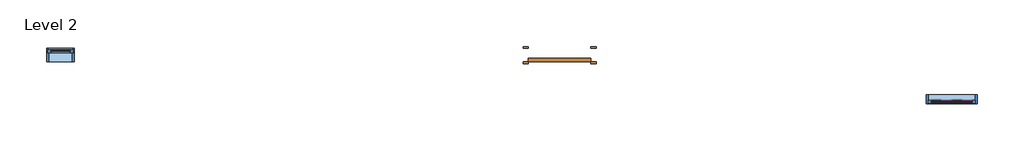
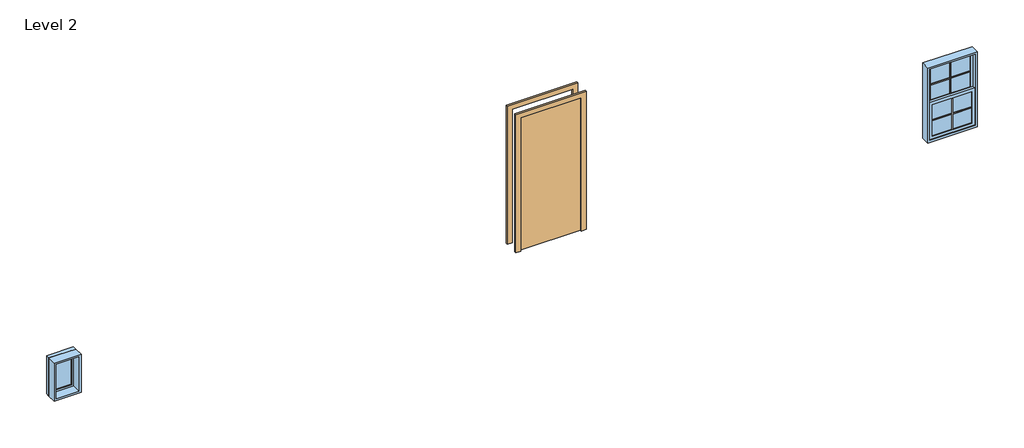
# One storey: 2 proxies, 2 windows, 1 door.
"""IFC4 building model written with IfcOpenShell, lengths in millimetres."""

import ifcopenshell
import ifcopenshell.guid

model = None  # the IFC model being written
_history = None  # IfcOwnerHistory: only IFC2X3 demands one
_inside = {}  # id of a spatial element -> (the spatial element, [elements in it])
_under = {}  # id of a project, library or spatial element -> (it, [spatial elements below it])
_declared = {}  # id of a project -> (the project, [libraries it declares])
_typed = {}  # id of a type object -> (the type object, [elements of that type])
_made_of = {}  # id of a material, layer set ... -> (it, [elements and type objects made of it])


def new_model(schema):
    """Start an empty IFC model of exactly this schema.

    Asked for "IFC4X3", IfcOpenShell would pick the latest addendum, in which some entities
    have other attributes; the version numbers below select the first issue.
    IFC2X3 requires an IfcOwnerHistory on every rooted entity: one is made here for all.
    """
    global model, _history
    if schema == "IFC4X3":
        model = ifcopenshell.file(schema_version=(4, 3, 0, 0))
    else:
        model = ifcopenshell.file(schema=schema)
    _inside.clear()
    _under.clear()
    _declared.clear()
    _typed.clear()
    _made_of.clear()
    _history = None
    if model.schema == "IFC2X3":
        org = make("IfcOrganization", Name="unknown")
        user = make(
            "IfcPersonAndOrganization",
            ThePerson=make("IfcPerson", FamilyName="unknown"),
            TheOrganization=org,
        )
        app = make(
            "IfcApplication",
            ApplicationDeveloper=org,
            Version="unknown",
            ApplicationFullName="unknown",
            ApplicationIdentifier="unknown",
        )
        _history = make(
            "IfcOwnerHistory",
            OwningUser=user,
            OwningApplication=app,
            ChangeAction="ADDED",
            CreationDate=0,
        )
    return model


def make(cls, **values):
    """One entity of the class cls with the attributes given. An attribute that is None is left unset."""
    return model.create_entity(
        cls, **{name: value for name, value in values.items() if value is not None}
    )


def rooted(cls, **values):
    """An entity with a GlobalId (a new one), such as an element, a storey or a relation."""
    return make(cls, GlobalId=ifcopenshell.guid.new(), OwnerHistory=_history, **values)


def si_unit(unit_type, name, prefix=None):
    """IfcSIUnit, for example si_unit("LENGTHUNIT", "METRE", prefix="MILLI")."""
    return make("IfcSIUnit", UnitType=unit_type, Prefix=prefix, Name=name)


def assignment(units):
    """IfcUnitAssignment: the units of a project."""
    return None if units is None else make("IfcUnitAssignment", Units=units)


def point(xyz):
    """IfcCartesianPoint."""
    return None if xyz is None else make("IfcCartesianPoint", Coordinates=xyz)


def direction(xyz):
    """IfcDirection."""
    return None if xyz is None else make("IfcDirection", DirectionRatios=xyz)


def frame(location, z_axis=None, x_axis=None):
    """IfcAxis2Placement3D, a coordinate frame: its origin and axes. An axis left out is left unset."""
    return make(
        "IfcAxis2Placement3D",
        Location=point(location),
        Axis=direction(z_axis),
        RefDirection=direction(x_axis),
    )


def origin():
    """The frame at (0, 0, 0) with its axes left unset."""
    return frame((0.0, 0.0, 0.0))


def origin_with_axes():
    """The frame at (0, 0, 0) with the z axis (0, 0, 1) and the x axis (1, 0, 0) written out."""
    return frame((0.0, 0.0, 0.0), z_axis=(0.0, 0.0, 1.0), x_axis=(1.0, 0.0, 0.0))


def place(relative_to, where):
    """IfcLocalPlacement: puts the frame where relative to a parent placement (None: the world)."""
    return make(
        "IfcLocalPlacement", PlacementRelTo=relative_to, RelativePlacement=where
    )


def context(
    kind, dimensions, precision=None, world=None, true_north=None, identifier=None
):
    """IfcGeometricRepresentationContext, for example the 3D "Model" context."""
    return make(
        "IfcGeometricRepresentationContext",
        ContextIdentifier=identifier,
        ContextType=kind,
        CoordinateSpaceDimension=dimensions,
        Precision=precision,
        WorldCoordinateSystem=world,
        TrueNorth=true_north,
    )


def project(units=None, contexts=None):
    """IfcProject with its units and contexts."""
    return rooted(
        "IfcProject",
        Name="project",
        RepresentationContexts=contexts,
        UnitsInContext=assignment(units),
    )


def spatial(cls, under=None, at=None, **own):
    """A site, building, storey or space (cls), placed at a placement, below another one or the project."""
    s = rooted(cls, ObjectPlacement=at, **own)
    if under is not None:
        _under.setdefault(under.id(), (under, []))[1].append(s)
    return s


def polyline(points):
    """IfcPolyline through the points."""
    return make("IfcPolyline", Points=[point(p) for p in points])


def outline(outer, holes=None, kind="AREA"):
    """IfcArbitraryClosedProfileDef: a profile drawn as a closed curve; with holes, ...WithVoids."""
    if holes is None:
        return make("IfcArbitraryClosedProfileDef", ProfileType=kind, OuterCurve=outer)
    return make(
        "IfcArbitraryProfileDefWithVoids",
        ProfileType=kind,
        OuterCurve=outer,
        InnerCurves=holes,
    )


def extrude(swept, where, along, depth):
    """IfcExtrudedAreaSolid: the profile swept, set in the frame where, extruded along a direction by depth."""
    return make(
        "IfcExtrudedAreaSolid",
        SweptArea=swept,
        Position=where,
        ExtrudedDirection=direction(along),
        Depth=depth,
    )


def shape(context_of_items, identifier, shape_type, items):
    """IfcShapeRepresentation: the items that make up one representation, for example the "Body"."""
    return make(
        "IfcShapeRepresentation",
        ContextOfItems=context_of_items,
        RepresentationIdentifier=identifier,
        RepresentationType=shape_type,
        Items=items,
    )


def source(mapping_origin, context_of_items, identifier, shape_type, items):
    """IfcRepresentationMap: a shape defined once, which mapped items show again and again."""
    return make(
        "IfcRepresentationMap",
        MappingOrigin=mapping_origin,
        MappedRepresentation=shape(context_of_items, identifier, shape_type, items),
    )


def transform(
    local_origin,
    x_axis=None,
    y_axis=None,
    z_axis=None,
    scale=None,
    scale2=None,
    scale3=None,
    uniform=True,
):
    """IfcCartesianTransformationOperator3D, or its non-uniform kind. x_axis, y_axis, z_axis: its Axis1, 2, 3."""
    if uniform:
        return make(
            "IfcCartesianTransformationOperator3D",
            Axis1=direction(x_axis),
            Axis2=direction(y_axis),
            LocalOrigin=point(local_origin),
            Scale=scale,
            Axis3=direction(z_axis),
        )
    return make(
        "IfcCartesianTransformationOperator3DnonUniform",
        Axis1=direction(x_axis),
        Axis2=direction(y_axis),
        LocalOrigin=point(local_origin),
        Scale=scale,
        Axis3=direction(z_axis),
        Scale2=scale2,
        Scale3=scale3,
    )


def mapped(mapping_source, mapping_target):
    """IfcMappedItem: shows the shape of a source again, moved by a transform."""
    return make(
        "IfcMappedItem", MappingSource=mapping_source, MappingTarget=mapping_target
    )


def made_of(thing, what):
    """Note that an element or type object is made of a material, layer set ...; save() writes the relation."""
    if what is not None:
        _made_of.setdefault(what.id(), (what, []))[1].append(thing)
    return thing


def element(
    cls,
    number,
    at=None,
    inside=None,
    cuts=None,
    type_object=None,
    material=None,
    context=None,
    identifier="Body",
    shape_type=None,
    held_by="IfcProductDefinitionShape",
    body=None,
    shapes=None,
    **own,
):
    """One element of the class cls, such as IfcWall. Its Tag is "e" and its number.

    at: its placement. inside: the storey or other place that contains it. cuts: it is an
    opening in that element (IfcRelVoidsElement). A single representation is given by context,
    identifier, shape_type and body (its items); several are given by shapes. held_by: the class
    of the entity that holds the representations. save() writes the other relations.
    """
    e = rooted(cls, Tag="e%d" % number, ObjectPlacement=at, **own)
    if body is not None:
        shapes = [shape(context, identifier, shape_type, body)]
    if shapes is not None:
        e.Representation = make(held_by, Representations=shapes)
    if inside is not None:
        _inside.setdefault(inside.id(), (inside, []))[1].append(e)
    if cuts is not None:
        rooted(
            "IfcRelVoidsElement", RelatingBuildingElement=cuts, RelatedOpeningElement=e
        )
    if type_object is not None:
        _typed.setdefault(type_object.id(), (type_object, []))[1].append(e)
    return made_of(e, material)


def aggregate(whole, parts):
    """IfcRelAggregates: a whole, such as a stair, and the parts it consists of."""
    return rooted("IfcRelAggregates", RelatingObject=whole, RelatedObjects=parts)


def save(model, path):
    """Write the relations noted so far, then the file.

    IfcRelAggregates (storeys below a building ...), IfcRelContainedInSpatialStructure (elements
    in a storey), IfcRelDefinesByType, IfcRelAssociatesMaterial and IfcRelDeclares: one each for
    every whole, place, type object, material and project.
    """
    for whole, parts in _under.values():
        aggregate(whole, parts)
    for where, things in _inside.values():
        rooted(
            "IfcRelContainedInSpatialStructure",
            RelatedElements=things,
            RelatingStructure=where,
        )
    for kind, things in _typed.values():
        rooted("IfcRelDefinesByType", RelatedObjects=things, RelatingType=kind)
    for what, things in _made_of.values():
        rooted("IfcRelAssociatesMaterial", RelatedObjects=things, RelatingMaterial=what)
    for by, libraries in _declared.values():
        rooted("IfcRelDeclares", RelatingContext=by, RelatedDefinitions=libraries)
    model.write(path)


def m_muntin_pattern_2x2_m_muntin_pattern_2x2_aaec3afb(model_context):
    return source(origin(), model_context, "Body", "SweptSolid", [
        extrude(outline(polyline([(257.1375, -6.35), (257.1375, -298.8), (244.4375, -298.8), (244.4375, -6.35), (0.0, -6.35), (0.0, 6.35), (244.4375, 6.35), (244.4375, 298.8), (257.1375, 298.8), (257.1375, 6.35), (501.575, 6.35), (501.575, -6.35), (257.1375, -6.35)])), frame((0.0, 9.525, 0.0), z_axis=(0.0, 1.0, 0.0), x_axis=(0.0, 0.0, 1.0)), (0.0, 0.0, 1.0), 12.7),
        extrude(outline(polyline([(257.1375, -6.35), (257.1375, -298.8), (244.4375, -298.8), (244.4375, -6.35), (0.0, -6.35), (0.0, 6.35), (244.4375, 6.35), (244.4375, 298.8), (257.1375, 298.8), (257.1375, 6.35), (501.575, 6.35), (501.575, -6.35), (257.1375, -6.35)])), frame((0.0, -22.225, 0.0), z_axis=(0.0, 1.0, 0.0), x_axis=(0.0, 0.0, 1.0)), (0.0, 0.0, 1.0), 12.7),
    ])


def m_single_flush_0915_x_2134mm_6a9e8738(model_context):
    return source(origin(), model_context, "Body", "SweptSolid", [
        extrude(outline(polyline([(2210.0, -533.5), (0.0, -533.5), (0.0, -457.5), (2134.0, -457.5), (2134.0, 457.5), (0.0, 457.5), (0.0, 533.5), (2210.0, 533.5), (2210.0, -533.5)])), frame((0.0, 100.0, 0.0), z_axis=(0.0, 1.0, 0.0), x_axis=(0.0, 0.0, 1.0)), (0.0, 0.0, 1.0), 25.0),
        extrude(outline(polyline([(2210.0, 533.5), (2210.0, -533.5), (0.0, -533.5), (0.0, -457.5), (2134.0, -457.5), (2134.0, 457.5), (0.0, 457.5), (0.0, 533.5), (2210.0, 533.5)])), frame((0.0, -125.0, 0.0), z_axis=(0.0, 1.0, 0.0), x_axis=(0.0, 0.0, 1.0)), (0.0, 0.0, 1.0), 25.0),
        extrude(outline(polyline([(457.5, 49.0), (-457.5, 49.0), (-457.5, 100.0), (457.5, 100.0), (457.5, 49.0)])), origin_with_axes(), (0.0, 0.0, 1.0), 2134.0),
    ])


def m_fixed_0406_x_0610mm_8205b201(model_context):
    return source(origin(), model_context, "Body", "SweptSolid", [
        extrude(outline(polyline([(-140.0, 78.0), (140.0, 78.0), (140.0, 66.0), (-140.0, 66.0), (-140.0, 78.0)])), frame((0.0, 0.0, 978.0), z_axis=(0.0, 0.0, 1.0), x_axis=(1.0, 0.0, 0.0)), (0.0, 0.0, 1.0), 484.0),
        extrude(outline(polyline([(1506.0, -184.0), (934.0, -184.0), (934.0, 184.0), (1506.0, 184.0), (1506.0, -184.0)]), holes=[polyline([(1462.0, -140.0), (1462.0, 140.0), (978.0, 140.0), (978.0, -140.0), (1462.0, -140.0)])]), frame((0.0, 50.0, 0.0), z_axis=(0.0, 1.0, 0.0), x_axis=(0.0, 0.0, 1.0)), (0.0, 0.0, 1.0), 44.0),
        extrude(outline(polyline([(1525.0, -203.0), (915.0, -203.0), (915.0, 203.0), (1525.0, 203.0), (1525.0, -203.0)]), holes=[polyline([(1506.0, -184.0), (1506.0, 184.0), (934.0, 184.0), (934.0, -184.0), (1506.0, -184.0)])]), frame((0.0, 50.0, 0.0), z_axis=(0.0, 1.0, 0.0), x_axis=(0.0, 0.0, 1.0)), (0.0, 0.0, 1.0), 63.0),
        extrude(outline(polyline([(1525.0, -203.0), (915.0, -203.0), (915.0, 203.0), (1525.0, 203.0), (1525.0, -203.0)]), holes=[polyline([(1493.0, -171.0), (1493.0, 171.0), (947.0, 171.0), (947.0, -171.0), (1493.0, -171.0)])]), frame((0.0, -87.0, 0.0), z_axis=(0.0, 1.0, 0.0), x_axis=(0.0, 0.0, 1.0)), (0.0, 0.0, 1.0), 137.0),
    ])


def m_window_double_hung_750_x_1200mm_e7ea5f28(model_context):
    return source(origin(), model_context, "Body", "SweptSolid", [
        extrude(outline(polyline([(298.8, -669.85), (298.8, -676.2), (-298.8, -676.2), (-298.8, -669.85), (298.8, -669.85)])), frame((0.0, 0.0, 990.6), z_axis=(0.0, 0.0, 1.0), x_axis=(1.0, 0.0, 0.0)), (0.0, 0.0, 1.0), 501.575),
        extrude(outline(polyline([(-298.8, -682.55), (298.8, -682.55), (298.8, -688.9), (-298.8, -688.9), (-298.8, -682.55)])), frame((0.0, 0.0, 990.6), z_axis=(0.0, 0.0, 1.0), x_axis=(1.0, 0.0, 0.0)), (0.0, 0.0, 1.0), 501.575),
        extrude(outline(polyline([(298.8, -625.4), (298.8, -631.75), (-298.8, -631.75), (-298.8, -625.4), (298.8, -625.4)])), frame((0.0, 0.0, 1536.625), z_axis=(0.0, 0.0, 1.0), x_axis=(1.0, 0.0, 0.0)), (0.0, 0.0, 1.0), 501.575),
        extrude(outline(polyline([(-298.8, -638.1), (298.8, -638.1), (298.8, -644.45), (-298.8, -644.45), (-298.8, -638.1)])), frame((0.0, 0.0, 1536.625), z_axis=(0.0, 0.0, 1.0), x_axis=(1.0, 0.0, 0.0)), (0.0, 0.0, 1.0), 501.575),
        extrude(outline(polyline([(1536.625, -343.25), (946.15, -343.25), (946.15, 343.25), (1536.625, 343.25), (1536.625, -343.25)]), holes=[polyline([(1492.175, 298.8), (990.6, 298.8), (990.6, -298.8), (1492.175, -298.8), (1492.175, 298.8)])]), frame((0.0, -701.6, 0.0), z_axis=(0.0, 1.0, 0.0), x_axis=(0.0, 0.0, 1.0)), (0.0, 0.0, 1.0), 44.45),
        extrude(outline(polyline([(2082.65, -343.25), (1492.175, -343.25), (1492.175, 343.25), (2082.65, 343.25), (2082.65, -343.25)]), holes=[polyline([(2038.2, 298.8), (1536.625, 298.8), (1536.625, -298.8), (2038.2, -298.8), (2038.2, 298.8)])]), frame((0.0, -657.15, 0.0), z_axis=(0.0, 1.0, 0.0), x_axis=(0.0, 0.0, 1.0)), (0.0, 0.0, 1.0), 44.45),
        extrude(outline(polyline([(2114.4, -375.0), (914.4, -375.0), (914.4, 375.0), (2114.4, 375.0), (2114.4, -375.0)]), holes=[polyline([(2082.65, 343.25), (946.15, 343.25), (946.15, -343.25), (2082.65, -343.25), (2082.65, 343.25)])]), frame((0.0, -714.3, 0.0), z_axis=(0.0, 1.0, 0.0), x_axis=(0.0, 0.0, 1.0)), (0.0, 0.0, 1.0), 133.35),
    ])


model = new_model("IFC4")

# Units and contexts
model_context = context("Model", 3, world=origin())
ifc_project = project(units=[si_unit("LENGTHUNIT", "METRE", prefix="MILLI")], contexts=[model_context])

# Site, building, storey
site = spatial("IfcSite", under=ifc_project)
building = spatial("IfcBuilding", under=site)
storey = spatial("IfcBuildingStorey", under=building, Name="Level 2", Elevation=4000.0)

# Proxies
placement = place(None, origin())
m_muntin_pattern_2x2_m_muntin_pattern_2x2_shape = m_muntin_pattern_2x2_m_muntin_pattern_2x2_aaec3afb(model_context)
element("IfcBuildingElementProxy", 1, Name="M_Muntin Pattern_2x2 : M_Muntin Pattern_2x2", ObjectType="M_Muntin Pattern_2x2 : M_Muntin Pattern_2x2", at=placement, inside=storey, context=model_context, shape_type="MappedRepresentation", body=[
    mapped(m_muntin_pattern_2x2_m_muntin_pattern_2x2_shape, transform((-15264.9853759, 1399.5505832, 5536.625), x_axis=(1.0, 0.0, 0.0), y_axis=(0.0, 1.0, 0.0), z_axis=(0.0, 0.0, 1.0))),
])
element("IfcBuildingElementProxy", 2, Name="M_Muntin Pattern_2x2 : M_Muntin Pattern_2x2", ObjectType="M_Muntin Pattern_2x2 : M_Muntin Pattern_2x2", at=placement, inside=storey, context=model_context, shape_type="MappedRepresentation", body=[
    mapped(m_muntin_pattern_2x2_m_muntin_pattern_2x2_shape, transform((-15264.9853759, 1355.1005832, 4990.6), x_axis=(1.0, 0.0, 0.0), y_axis=(0.0, 1.0, 0.0), z_axis=(0.0, 0.0, 1.0))),
])

# Door
m_single_flush_0915_x_2134mm_shape = m_single_flush_0915_x_2134mm_6a9e8738(model_context)
element("IfcDoor", 3, ObjectType="M_Single-Flush : 0915 x 2134mm", at=placement, inside=storey, context=model_context, shape_type="MappedRepresentation", body=[
    mapped(m_single_flush_0915_x_2134mm_shape, transform((-20997.4853759, 2034.4755832, 4866.0), x_axis=(-1.0, 0.0, 0.0), y_axis=(0.0, -1.0, 0.0), z_axis=(0.0, 0.0, 1.0))),
])

# Windows
m_fixed_0406_x_0610mm_shape = m_fixed_0406_x_0610mm_8205b201(model_context)
element("IfcWindow", 4, ObjectType="M_Fixed : 0406 x 0610mm", at=placement, inside=storey, context=model_context, shape_type="MappedRepresentation", body=[
    mapped(m_fixed_0406_x_0610mm_shape, transform((-28293.5284847, 2021.4755832, 4000.0), x_axis=(1.0, 0.0, 0.0), y_axis=(0.0, 1.0, 0.0), z_axis=(0.0, 0.0, 1.0))),
])
m_window_double_hung_750_x_1200mm_shape = m_window_double_hung_750_x_1200mm_e7ea5f28(model_context)
element("IfcWindow", 5, ObjectType="M_Window-Double-Hung : 750 x 1200mm", at=placement, inside=storey, context=model_context, shape_type="MappedRepresentation", body=[
    mapped(m_window_double_hung_750_x_1200mm_shape, transform((-15264.9853759, 2034.4755832, 4000.0), x_axis=(1.0, 0.0, 0.0), y_axis=(0.0, 1.0, 0.0), z_axis=(0.0, 0.0, 1.0))),
])

save(model, "model.ifc")

# Revit data of these elements
# Type "M_Muntin Pattern_2x2 : M_Muntin Pattern_2x2"
#   Width [instance default] = 1200 mm
#   Thickness = 12.7 mm
#   Height [instance default] = 1200 mm
#   Distance = 19.05 mm
#   Interior Material [instance default] = none
#   Exterior Material [instance default] = none
#   Default Elevation = 0
# Type "M_Single-Flush : 0915 x 2134mm"
#   Type Mark = "20"
#   Construction Type Id = "MDOOR"
#   Analytic Construction = "Metal"
#   Thickness = 51 mm
#   Thermal Resistance (R) = 0.270117 (m²·K)/W
#   Heat Transfer Coefficient (U) = 3.7021 W/(m²·K)
#   Height = 2134 mm
#   Trim Projection Ext = 25 mm
#   Trim Projection Int = 25 mm
#   Trim Width = 76 mm
#   Width = 915 mm
#   Define Thermal Properties by = 1
#   Define Thermal Properties by = 1
#   Door Material = Door - Panel
#   Frame Material = Door - Frame
#   Visual Light Transmittance = 0
#   Solar Heat Gain Coefficient = 0
#   Function = (empty or 0)
#   Wall Closure = (empty or 0)
# Type "M_Fixed : 0406 x 0610mm"
#   Type Mark = "10"
#   Construction Type Id = "GSP4R"
#   Analytic Construction = "1/8 in Pilkington single glazing"
#   Visual Light Transmittance = 0.9
#   Thermal Resistance (R) = 0.271106 (m²·K)/W
#   Solar Heat Gain Coefficient = 0.78
#   Heat Transfer Coefficient (U) = 3.6886 W/(m²·K)
#   Height = 610 mm
#   Default Sill Height = 915 mm
#   Width = 406 mm
#   Window Inset = 19 mm
#   Define Thermal Properties by = 1
#   Define Thermal Properties by = 1
#   Frame Exterior Material = Sash
#   Frame Interior Material = Sash
#   Glass Pane Material = Glass
#   Sash = Sash
#   Wall Closure = (empty or 0)
# Type "M_Window-Double-Hung : 750 x 1200mm"
#   Type Mark = "22"
#   Fire Rating = "0.5h"
#   Construction Type Id = "DG-DR"
#   Assembly Code = "B2020100"
#   Analytic Construction = "Double glazing - domestic"
#   Wall Thickness [instance default] = 150 mm
#   Window Inset [instance default] = 0 mm
#   Visual Light Transmittance = 0.81
#   Thermal Resistance (R) = 0.319569 (m²·K)/W
#   Solar Heat Gain Coefficient = 0.76
#   Muntin Width = 597.6 mm
#   Muntin Height = 501.575 mm
#   Interior Wall Closure [instance default] = 35.7 mm
#   Rough Width = 765 mm
#   Rough Height = 1215 mm
#   Frame Extension [instance default] = 31.75 mm
#   Exterior Wall Closure [instance default] = 12.7 mm
#   Extension Jamb [instance default] = 35.7 mm
#   Heat Transfer Coefficient (U) = 3.12929 W/(m²·K)
#   Height = 1200 mm
#   Width = 750 mm
#   Define Thermal Properties by = 1
#   Top Muntin Visibility = yes
#   Indicator Visibility [instance default] = yes
#   Extension Jamb Visibility [instance default] = yes
#   Interior Trim Visibility [instance default] = yes
#   Exterior Trim Visibility [instance default] = yes
#   Define Thermal Properties by = 1
#   Bottom Muntin Visibility = yes
#   Muntin Pattern = M_Muntin Pattern_2x2 : M_Muntin Pattern_2x2
#   Interior Trim Material = Wood - Stained
#   Interior Trim = M_Trim-Window-Interior-Flat : Picture Frame
#   Exterior Trim Material = Clad - White
#   Exterior Trim = M_Trim-Window-Exterior-Flat : with Sill
#   Glass Panel Material = Glass
#   Exterior Frame Material = Clad - White
#   Interior Frame Material = Wood - Stained
#   Wall Closure = (empty or 0)
# Elements 1, 2 (IfcBuildingElementProxy, "M_Muntin Pattern_2x2 : M_Muntin Pattern_2x2")
#   Width = 597.6 mm
#   Height = 501.575 mm
#   Interior Material = Wood - Stained
#   Exterior Material = Clad - White
#   Phase Created = New Construction
#   Materials on its faces: "Clad - White", "Wood - Stained"
# Element 3 (IfcDoor, "M_Single-Flush : 0915 x 2134mm")
#   SpeckleObjectUpdateDescription = "location change"
#   SpeckleObjectTestNumber = 5
#   Phase Created = New Construction
#   Materials on its faces: "Door - Frame", "Door - Panel"
# Element 4 (IfcWindow, "M_Fixed : 0406 x 0610mm")
#   Mark = "1"
#   SpeckleObjectUpdateDescription = "level change"
#   SpeckleObjectTestNumber = 2
#   Phase Created = New Construction
#   Materials on its faces: "Sash", "Glass"
# Element 5 (IfcWindow, "M_Window-Double-Hung : 750 x 1200mm")
#   Mark = "4"
#   SpeckleObjectUpdateDescription = "None yet"
#   Window Inset = 700 mm
#   Interior Wall Closure = 60 mm
#   Frame Extension = 31.75 mm
#   Exterior Wall Closure = 50 mm
#   SpeckleObjectTestNumber = 7
#   Interior Trim Visibility = no
#   Indicator Visibility = no
#   Exterior Trim Visibility = no
#   Phase Created = New Construction
#   Materials on its faces: "Wood - Stained", "Glass", "Clad - White"
# Materials
#   "Door - Panel": class "Wood", colour RGB 210 159 95, transparency 0, Cost = 0
#   "Door - Frame": class "Miscellaneous", colour RGB 118 70 51, transparency 0, Cost = 0
#   "Sash": class "Wood", colour RGB 224 178 126, transparency 0, Cost = 0
#   "Glass": class "Glass", colour RGB 0 128 192, transparency 0.9, Description = "Soda Lime Glass", Cost = 0
#   "Wood - Stained": class "Wood", colour RGB 224 178 126, transparency 0, Cost = 0
#   "Clad - White": class "Wood", colour RGB 242 242 238, transparency 0, Cost = 0
